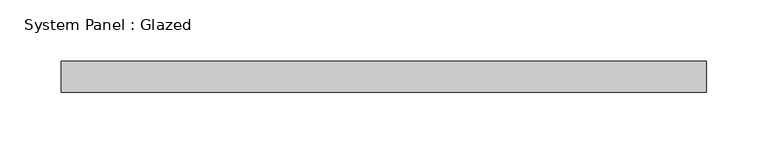
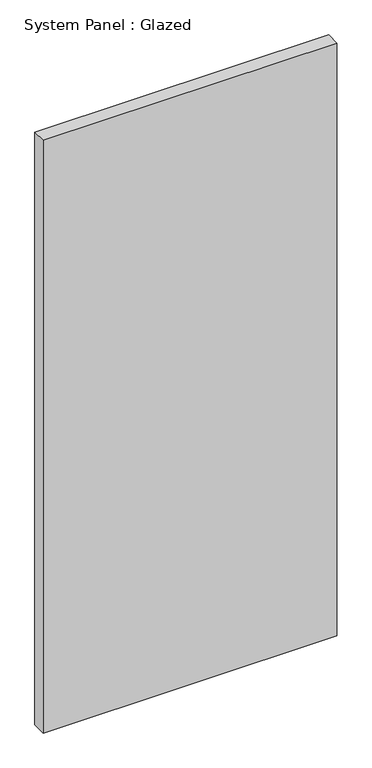
"""IFC4 building model written with IfcOpenShell, lengths in millimetres: plate geometry, System Panel : Glazed."""

from ifc_helpers import new_model, si_unit, origin, origin_with_axes, place, context, project, spatial, polyline, outline, extrude, source, transform, mapped, element, save


def system_panel_glazed_4b84483b(model_context):
    return source(origin(), model_context, "Body", "SweptSolid", [
        extrude(outline(polyline([(263.525, -44.45), (-263.525, -44.45), (-263.525, -19.05), (263.525, -19.05), (263.525, -44.45)])), origin_with_axes(), (0.0, 0.0, 1.0), 1123.95),
    ])


if __name__ == "__main__":
    model = new_model("IFC4")
    model_context = context("Model", 3, world=origin())
    ifc_project = project(units=[si_unit("LENGTHUNIT", "METRE", prefix="MILLI")], contexts=[model_context])
    site = spatial("IfcSite", under=ifc_project)
    building = spatial("IfcBuilding", under=site)
    placement = place(None, origin())
    system_panel_glazed_shape = system_panel_glazed_4b84483b(model_context)
    element("IfcPlate", 1, ObjectType="System Panel : Glazed", at=placement, inside=building, context=model_context, shape_type="MappedRepresentation", body=[
        mapped(system_panel_glazed_shape, transform((0.0, 0.0, 0.0), x_axis=(1.0, 0.0, 0.0), y_axis=(0.0, 1.0, 0.0), z_axis=(0.0, 0.0, 1.0))),
    ])
    save(model, "model.ifc")

# Revit data of these elements
# Element 1 (IfcPlate, "System Panel : Glazed")
#   Materials on its faces: "Glass"
# Materials
#   "Glass": class "Glass", colour RGB 0 128 192, transparency 0.75
